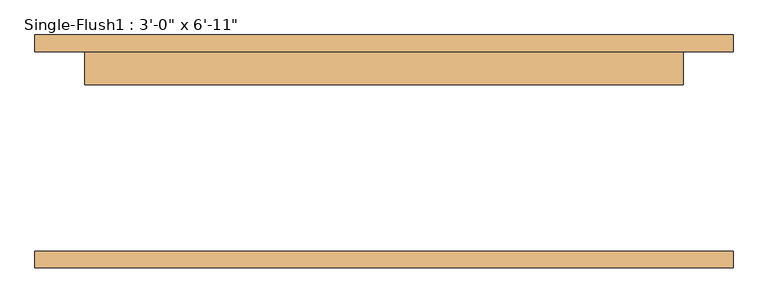
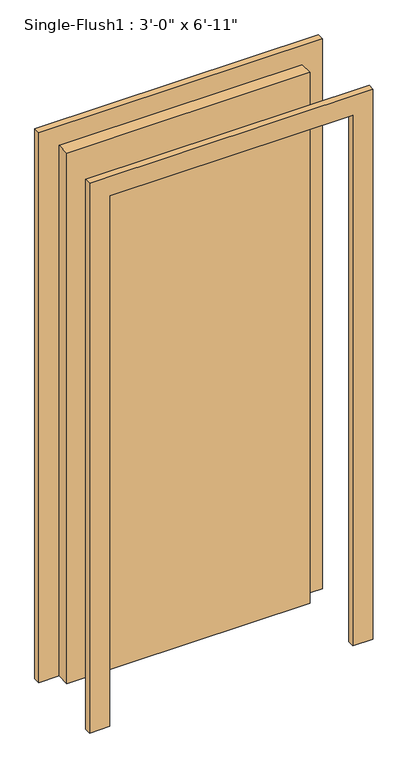
"""IFC4 building model written with IfcOpenShell, lengths in millimetres: door geometry."""

from ifc_helpers import new_model, si_unit, frame, origin, origin_with_axes, place, context, project, spatial, polyline, outline, extrude, source, transform, mapped, element, save


def door_a6ca3d0c(model_context):
    return source(origin(), model_context, "Body", "SweptSolid", [
        extrude(outline(polyline([(2184.4, -533.4), (0.0, -533.4), (0.0, -457.2), (2108.2, -457.2), (2108.2, 457.2), (0.0, 457.2), (0.0, 533.4), (2184.4, 533.4), (2184.4, -533.4)])), frame((0.0, 152.4, 0.0), z_axis=(0.0, 1.0, 0.0), x_axis=(0.0, 0.0, 1.0)), (0.0, 0.0, 1.0), 25.4),
        extrude(outline(polyline([(2184.4, 533.4), (2184.4, -533.4), (0.0, -533.4), (0.0, -457.2), (2108.2, -457.2), (2108.2, 457.2), (0.0, 457.2), (0.0, 533.4), (2184.4, 533.4)])), frame((0.0, -177.8, 0.0), z_axis=(0.0, 1.0, 0.0), x_axis=(0.0, 0.0, 1.0)), (0.0, 0.0, 1.0), 25.4),
        extrude(outline(polyline([(457.2, 101.6), (-457.2, 101.6), (-457.2, 152.4), (457.2, 152.4), (457.2, 101.6)])), origin_with_axes(), (0.0, 0.0, 1.0), 2108.2),
    ])


if __name__ == "__main__":
    model = new_model("IFC4")
    model_context = context("Model", 3, world=origin())
    ifc_project = project(units=[si_unit("LENGTHUNIT", "METRE", prefix="MILLI")], contexts=[model_context])
    site = spatial("IfcSite", under=ifc_project)
    building = spatial("IfcBuilding", under=site)
    placement = place(None, origin())
    door_shape = door_a6ca3d0c(model_context)
    element("IfcDoor", 1, ObjectType="Single-Flush1 : 3'-0\" x 6'-11\"", at=placement, inside=building, context=model_context, shape_type="MappedRepresentation", body=[
        mapped(door_shape, transform((0.0, 0.0, 0.0), x_axis=(1.0, 0.0, 0.0), y_axis=(0.0, 1.0, 0.0), z_axis=(0.0, 0.0, 1.0))),
    ])
    save(model, "model.ifc")

# Revit data of these elements
# Type "Single-Flush1 : 3'-0\" x 6'-11\""
#   Type Mark = "D3"
#   Construction Type Id = "MDOOR"
#   Assembly Code = "C1020"
#   Analytic Construction = "Metal"
#   Thickness = 0' - 2"
#   Heat Transfer Coefficient (U) = 3.7021 W/(m²·K)
#   Height = 6' - 11"
#   Trim Projection Ext = 0' - 1"
#   Trim Projection Int = 0' - 1"
#   Trim Width = 0' - 3"
#   Width = 3' - 0"
#   Door Material = Door - Panel
#   Frame Material = Door - Frame
#   Visual Light Transmittance = 0
#   Solar Heat Gain Coefficient = 0
#   Function = (empty or 0)
#   Wall Closure = (empty or 0)
# Element 1 (IfcDoor, "Single-Flush1 : 3'-0\" x 6'-11\"")
#   Materials on its faces: "Door - Frame", "Door - Panel"
# Materials
#   "Door - Panel": class "Wood", colour RGB 210 159 95, transparency 0, Cost = 0
#   "Door - Frame": class "Miscellaneous", colour RGB 118 70 51, transparency 0, Cost = 0
